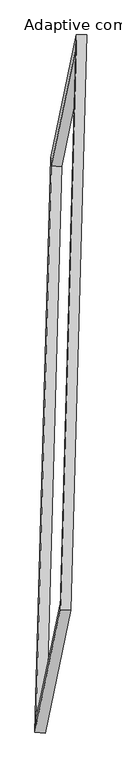
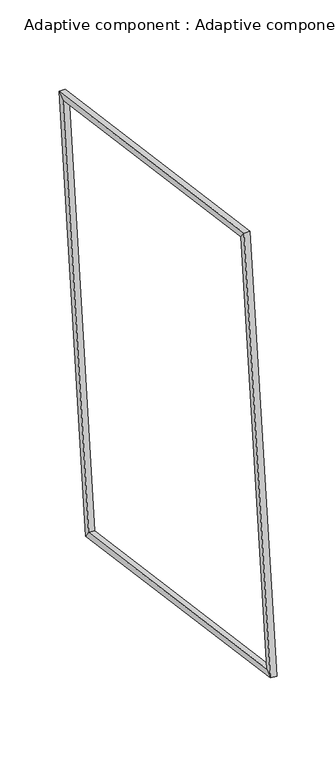
"""IFC4 building model written with IfcOpenShell, lengths in millimetres: proxy geometry, Adaptive component : Adaptive component."""

import ifcopenshell
import ifcopenshell.guid

model = None  # the IFC model being written
_history = None  # IfcOwnerHistory: only IFC2X3 demands one
_inside = {}  # id of a spatial element -> (the spatial element, [elements in it])
_under = {}  # id of a project, library or spatial element -> (it, [spatial elements below it])
_declared = {}  # id of a project -> (the project, [libraries it declares])
_typed = {}  # id of a type object -> (the type object, [elements of that type])
_made_of = {}  # id of a material, layer set ... -> (it, [elements and type objects made of it])


def new_model(schema):
    """Start an empty IFC model of exactly this schema.

    Asked for "IFC4X3", IfcOpenShell would pick the latest addendum, in which some entities
    have other attributes; the version numbers below select the first issue.
    IFC2X3 requires an IfcOwnerHistory on every rooted entity: one is made here for all.
    """
    global model, _history
    if schema == "IFC4X3":
        model = ifcopenshell.file(schema_version=(4, 3, 0, 0))
    else:
        model = ifcopenshell.file(schema=schema)
    _inside.clear()
    _under.clear()
    _declared.clear()
    _typed.clear()
    _made_of.clear()
    _history = None
    if model.schema == "IFC2X3":
        org = make("IfcOrganization", Name="unknown")
        user = make(
            "IfcPersonAndOrganization",
            ThePerson=make("IfcPerson", FamilyName="unknown"),
            TheOrganization=org,
        )
        app = make(
            "IfcApplication",
            ApplicationDeveloper=org,
            Version="unknown",
            ApplicationFullName="unknown",
            ApplicationIdentifier="unknown",
        )
        _history = make(
            "IfcOwnerHistory",
            OwningUser=user,
            OwningApplication=app,
            ChangeAction="ADDED",
            CreationDate=0,
        )
    return model


def make(cls, **values):
    """One entity of the class cls with the attributes given. An attribute that is None is left unset."""
    return model.create_entity(
        cls, **{name: value for name, value in values.items() if value is not None}
    )


def rooted(cls, **values):
    """An entity with a GlobalId (a new one), such as an element, a storey or a relation."""
    return make(cls, GlobalId=ifcopenshell.guid.new(), OwnerHistory=_history, **values)


def si_unit(unit_type, name, prefix=None):
    """IfcSIUnit, for example si_unit("LENGTHUNIT", "METRE", prefix="MILLI")."""
    return make("IfcSIUnit", UnitType=unit_type, Prefix=prefix, Name=name)


def assignment(units):
    """IfcUnitAssignment: the units of a project."""
    return None if units is None else make("IfcUnitAssignment", Units=units)


def point(xyz):
    """IfcCartesianPoint."""
    return None if xyz is None else make("IfcCartesianPoint", Coordinates=xyz)


def direction(xyz):
    """IfcDirection."""
    return None if xyz is None else make("IfcDirection", DirectionRatios=xyz)


def frame(location, z_axis=None, x_axis=None):
    """IfcAxis2Placement3D, a coordinate frame: its origin and axes. An axis left out is left unset."""
    return make(
        "IfcAxis2Placement3D",
        Location=point(location),
        Axis=direction(z_axis),
        RefDirection=direction(x_axis),
    )


def origin():
    """The frame at (0, 0, 0) with its axes left unset."""
    return frame((0.0, 0.0, 0.0))


def place(relative_to, where):
    """IfcLocalPlacement: puts the frame where relative to a parent placement (None: the world)."""
    return make(
        "IfcLocalPlacement", PlacementRelTo=relative_to, RelativePlacement=where
    )


def context(
    kind, dimensions, precision=None, world=None, true_north=None, identifier=None
):
    """IfcGeometricRepresentationContext, for example the 3D "Model" context."""
    return make(
        "IfcGeometricRepresentationContext",
        ContextIdentifier=identifier,
        ContextType=kind,
        CoordinateSpaceDimension=dimensions,
        Precision=precision,
        WorldCoordinateSystem=world,
        TrueNorth=true_north,
    )


def project(units=None, contexts=None):
    """IfcProject with its units and contexts."""
    return rooted(
        "IfcProject",
        Name="project",
        RepresentationContexts=contexts,
        UnitsInContext=assignment(units),
    )


def spatial(cls, under=None, at=None, **own):
    """A site, building, storey or space (cls), placed at a placement, below another one or the project."""
    s = rooted(cls, ObjectPlacement=at, **own)
    if under is not None:
        _under.setdefault(under.id(), (under, []))[1].append(s)
    return s


def faces_of(points, faces, orient=None, outer=None):
    """IfcFace entities. A face is a list of loops; a loop is a list of indices into points, from 0.

    orient and outer hold one flag for each loop. By default every Orientation is true, the
    first loop of a face is its IfcFaceOuterBound and the others are IfcFaceBound.
    """
    made = []
    for i, loops in enumerate(faces):
        bounds = []
        for j, loop in enumerate(loops):
            is_outer = j == 0 if outer is None else outer[i][j]
            bounds.append(
                make(
                    "IfcFaceOuterBound" if is_outer else "IfcFaceBound",
                    Bound=make("IfcPolyLoop", Polygon=[points[k] for k in loop]),
                    Orientation=True if orient is None else orient[i][j],
                )
            )
        made.append(make("IfcFace", Bounds=bounds))
    return made


def faceted_brep(points, faces, orient=None, outer=None, voids=None):
    """IfcFacetedBrep: a solid bounded by flat faces; with voids (closed shells), ...WithVoids."""
    shared = [point(p) for p in points]
    hull = make("IfcClosedShell", CfsFaces=faces_of(shared, faces, orient, outer))
    if voids is None:
        return make("IfcFacetedBrep", Outer=hull)
    return make(
        "IfcFacetedBrepWithVoids",
        Outer=hull,
        Voids=[
            make(cls, CfsFaces=faces_of(shared, fs, o, b)) for cls, fs, o, b in voids
        ],
    )


def shape(context_of_items, identifier, shape_type, items):
    """IfcShapeRepresentation: the items that make up one representation, for example the "Body"."""
    return make(
        "IfcShapeRepresentation",
        ContextOfItems=context_of_items,
        RepresentationIdentifier=identifier,
        RepresentationType=shape_type,
        Items=items,
    )


def source(mapping_origin, context_of_items, identifier, shape_type, items):
    """IfcRepresentationMap: a shape defined once, which mapped items show again and again."""
    return make(
        "IfcRepresentationMap",
        MappingOrigin=mapping_origin,
        MappedRepresentation=shape(context_of_items, identifier, shape_type, items),
    )


def transform(
    local_origin,
    x_axis=None,
    y_axis=None,
    z_axis=None,
    scale=None,
    scale2=None,
    scale3=None,
    uniform=True,
):
    """IfcCartesianTransformationOperator3D, or its non-uniform kind. x_axis, y_axis, z_axis: its Axis1, 2, 3."""
    if uniform:
        return make(
            "IfcCartesianTransformationOperator3D",
            Axis1=direction(x_axis),
            Axis2=direction(y_axis),
            LocalOrigin=point(local_origin),
            Scale=scale,
            Axis3=direction(z_axis),
        )
    return make(
        "IfcCartesianTransformationOperator3DnonUniform",
        Axis1=direction(x_axis),
        Axis2=direction(y_axis),
        LocalOrigin=point(local_origin),
        Scale=scale,
        Axis3=direction(z_axis),
        Scale2=scale2,
        Scale3=scale3,
    )


def mapped(mapping_source, mapping_target):
    """IfcMappedItem: shows the shape of a source again, moved by a transform."""
    return make(
        "IfcMappedItem", MappingSource=mapping_source, MappingTarget=mapping_target
    )


def made_of(thing, what):
    """Note that an element or type object is made of a material, layer set ...; save() writes the relation."""
    if what is not None:
        _made_of.setdefault(what.id(), (what, []))[1].append(thing)
    return thing


def element(
    cls,
    number,
    at=None,
    inside=None,
    cuts=None,
    type_object=None,
    material=None,
    context=None,
    identifier="Body",
    shape_type=None,
    held_by="IfcProductDefinitionShape",
    body=None,
    shapes=None,
    **own,
):
    """One element of the class cls, such as IfcWall. Its Tag is "e" and its number.

    at: its placement. inside: the storey or other place that contains it. cuts: it is an
    opening in that element (IfcRelVoidsElement). A single representation is given by context,
    identifier, shape_type and body (its items); several are given by shapes. held_by: the class
    of the entity that holds the representations. save() writes the other relations.
    """
    e = rooted(cls, Tag="e%d" % number, ObjectPlacement=at, **own)
    if body is not None:
        shapes = [shape(context, identifier, shape_type, body)]
    if shapes is not None:
        e.Representation = make(held_by, Representations=shapes)
    if inside is not None:
        _inside.setdefault(inside.id(), (inside, []))[1].append(e)
    if cuts is not None:
        rooted(
            "IfcRelVoidsElement", RelatingBuildingElement=cuts, RelatedOpeningElement=e
        )
    if type_object is not None:
        _typed.setdefault(type_object.id(), (type_object, []))[1].append(e)
    return made_of(e, material)


def aggregate(whole, parts):
    """IfcRelAggregates: a whole, such as a stair, and the parts it consists of."""
    return rooted("IfcRelAggregates", RelatingObject=whole, RelatedObjects=parts)


def save(model, path):
    """Write the relations noted so far, then the file.

    IfcRelAggregates (storeys below a building ...), IfcRelContainedInSpatialStructure (elements
    in a storey), IfcRelDefinesByType, IfcRelAssociatesMaterial and IfcRelDeclares: one each for
    every whole, place, type object, material and project.
    """
    for whole, parts in _under.values():
        aggregate(whole, parts)
    for where, things in _inside.values():
        rooted(
            "IfcRelContainedInSpatialStructure",
            RelatedElements=things,
            RelatingStructure=where,
        )
    for kind, things in _typed.values():
        rooted("IfcRelDefinesByType", RelatedObjects=things, RelatingType=kind)
    for what, things in _made_of.values():
        rooted("IfcRelAssociatesMaterial", RelatedObjects=things, RelatingMaterial=what)
    for by, libraries in _declared.values():
        rooted("IfcRelDeclares", RelatingContext=by, RelatedDefinitions=libraries)
    model.write(path)


def adaptive_component_adaptive_component_f6ad3491(model_context):
    return source(origin(), model_context, "Body", "Brep", [
        faceted_brep([(107.1639723, 1750.3366168, 3279.9532791), (172.1858768, 1750.2373374, 3279.4524243), (13.0911406, 986.8884768, -1203.7952408), (-51.8074771, 987.5792953, -1199.8201994), (104.8785089, 1675.3592486, 3226.8490219), (-49.5496004, 934.401225, -1124.8943289), (169.9004134, 1675.2599691, 3226.3481672), (15.3490174, 933.7104065, -1128.8693703), (-86.1754603, -2592.9522312, -590.7440946), (-150.977734, -2588.7869658, -587.3640556), (-145.169401, -2513.9253189, -534.3651092), (-80.3671274, -2518.0905843, -537.7451482), (72.9192759, -1829.6033706, 3892.5035705), (7.9937155, -1826.0296443, 3892.4094229), (9.2587082, -1772.9672954, 3817.3782417), (74.1842686, -1776.5410217, 3817.4723893)], [[[0, 1, 2, 3]], [[4, 0, 3, 5]], [[6, 4, 5, 7]], [[1, 6, 7, 2]], [[3, 2, 8, 9]], [[5, 3, 9, 10]], [[7, 5, 10, 11]], [[2, 7, 11, 8]], [[9, 8, 12, 13]], [[10, 9, 13, 14]], [[11, 10, 14, 15]], [[8, 11, 15, 12]], [[13, 12, 1, 0]], [[14, 13, 0, 4]], [[15, 14, 4, 6]], [[12, 15, 6, 1]]]),
    ])


if __name__ == "__main__":
    model = new_model("IFC4")
    model_context = context("Model", 3, world=origin())
    ifc_project = project(units=[si_unit("LENGTHUNIT", "METRE", prefix="MILLI")], contexts=[model_context])
    site = spatial("IfcSite", under=ifc_project)
    building = spatial("IfcBuilding", under=site)
    placement = place(None, origin())
    adaptive_component_adaptive_component_shape = adaptive_component_adaptive_component_f6ad3491(model_context)
    element("IfcBuildingElementProxy", 1, Name="Adaptive component : Adaptive component", ObjectType="Adaptive component : Adaptive component", at=placement, inside=building, context=model_context, shape_type="MappedRepresentation", body=[
        mapped(adaptive_component_adaptive_component_shape, transform((0.0, 0.0, 0.0), x_axis=(1.0, 0.0, 0.0), y_axis=(0.0, 1.0, 0.0), z_axis=(0.0, 0.0, 1.0))),
    ])
    save(model, "model.ifc")

# Revit data of these elements
# Type "Adaptive component : Adaptive component"
#   r [instance default] = 2063.125 mm
#   2r [instance default] = 4126.251 mm
#   Number [instance default] = 5
#   Default Elevation = 0
# Element 1 (IfcBuildingElementProxy, "Adaptive component : Adaptive component")
#   r = 2817.89 mm
#   2r = 5635.78 mm
#   Number = 31
